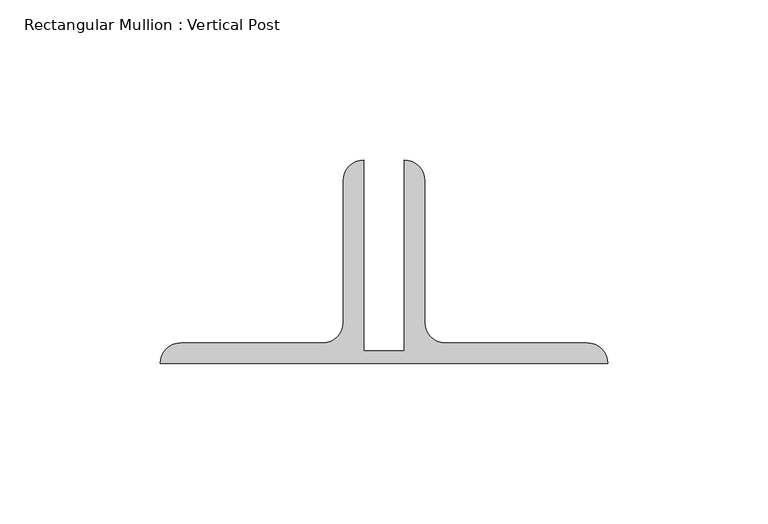
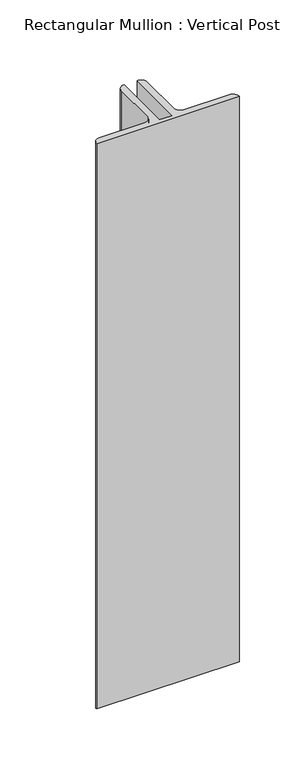
"""IFC4 building model written with IfcOpenShell, lengths in millimetres: member geometry, Rectangular Mullion : Vertical Post."""

from ifc_helpers import new_model, si_unit, point, frame, frame_2d, origin, place, context, project, spatial, polyline, circle_curve, trimmed, segment, composite_curve, outline, extrude, source, transform, mapped, element, save


def rectangular_mullion_vertical_post_29492a09(model_context):
    return source(origin(), model_context, "Body", "SweptSolid", [
        extrude(outline(composite_curve([segment(polyline([(-6.35, 22.9145205), (6.35, 22.9145205), (6.35, 82.55)]), True, "CONTINUOUS"), segment(trimmed(circle_curve(frame_2d((6.35, 76.2)), 6.35), [point((6.35, 82.55))], [point((12.7, 76.2))], False, "CARTESIAN"), True, "CONTINUOUS"), segment(polyline([(12.7, 76.2), (12.7, 31.75)]), True, "CONTINUOUS"), segment(trimmed(circle_curve(frame_2d((19.05, 31.75)), 6.35), [point((12.7, 31.75))], [point((19.05, 25.4))], True, "CARTESIAN"), True, "CONTINUOUS"), segment(polyline([(19.05, 25.4), (63.5, 25.4)]), True, "CONTINUOUS"), segment(trimmed(circle_curve(frame_2d((63.5, 19.05)), 6.35), [point((63.5, 25.4))], [point((69.85, 19.05))], False, "CARTESIAN"), True, "CONTINUOUS"), segment(polyline([(69.85, 19.05), (-69.85, 19.05)]), True, "CONTINUOUS"), segment(trimmed(circle_curve(frame_2d((-63.5, 19.05)), 6.35), [point((-69.85, 19.05))], [point((-63.5, 25.4))], False, "CARTESIAN"), True, "CONTINUOUS"), segment(polyline([(-63.5, 25.4), (-19.05, 25.4)]), True, "CONTINUOUS"), segment(trimmed(circle_curve(frame_2d((-19.05, 31.75)), 6.35), [point((-19.05, 25.4))], [point((-12.7, 31.75))], True, "CARTESIAN"), True, "CONTINUOUS"), segment(polyline([(-12.7, 31.75), (-12.7, 76.2)]), True, "CONTINUOUS"), segment(trimmed(circle_curve(frame_2d((-6.35, 76.2)), 6.35), [point((-12.7, 76.2))], [point((-6.35, 82.55))], False, "CARTESIAN"), True, "CONTINUOUS"), segment(polyline([(-6.35, 82.55), (-6.35, 22.9145205)]), True, "CONTINUOUS")], self_intersect=False)), frame((0.0, 0.0, -584.2), z_axis=(0.0, 0.0, 1.0), x_axis=(1.0, 0.0, 0.0)), (0.0, 0.0, 1.0), 584.2),
    ])


if __name__ == "__main__":
    model = new_model("IFC4")
    model_context = context("Model", 3, world=origin())
    ifc_project = project(units=[si_unit("LENGTHUNIT", "METRE", prefix="MILLI")], contexts=[model_context])
    site = spatial("IfcSite", under=ifc_project)
    building = spatial("IfcBuilding", under=site)
    placement = place(None, origin())
    rectangular_mullion_vertical_post_shape = rectangular_mullion_vertical_post_29492a09(model_context)
    element("IfcMember", 1, ObjectType="Rectangular Mullion : Vertical Post", at=placement, inside=building, context=model_context, shape_type="MappedRepresentation", body=[
        mapped(rectangular_mullion_vertical_post_shape, transform((0.0, 0.0, 0.0), x_axis=(1.0, 0.0, 0.0), y_axis=(0.0, 1.0, 0.0), z_axis=(0.0, 0.0, 1.0))),
    ])
    save(model, "model.ifc")

# Revit data of these elements
# Type "Rectangular Mullion : Vertical Post"
#   built-in parameter 1007351 = -0.0625 (stored number, unit not read)
#   built-in parameter 1007322 = 0.0126789 (stored number, unit not read)
#   built-in parameter 1007321 = 0.229167 (stored number, unit not read)
#   built-in parameter 1007320 = 0.229167 (stored number, unit not read)
# Element 1 (IfcMember, "Rectangular Mullion : Vertical Post")
#   Materials on its faces: "GATE POST: GALVANIZED ANGLES"
# Materials
#   "GATE POST: GALVANIZED ANGLES": class "Unassigned", colour RGB 120 120 120, transparency 0, Cost = 0
